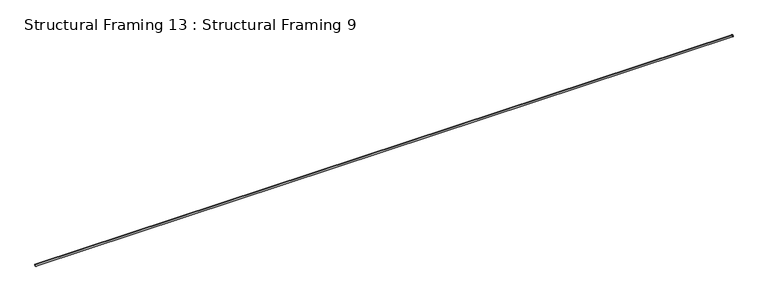
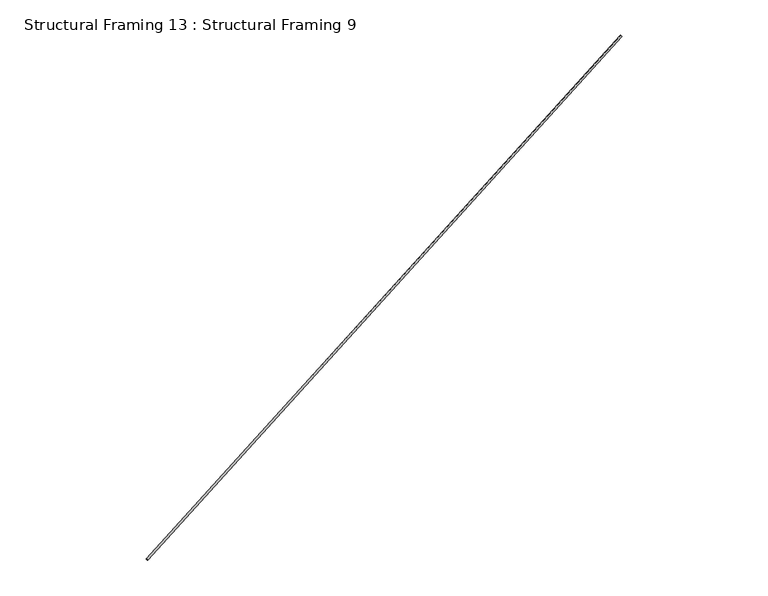
"""IFC4 building model written with IfcOpenShell, lengths in millimetres: beam geometry, Structural Framing 13 : Structural Framing 9."""

from ifc_helpers import new_model, si_unit, point, frame, origin, origin_2d, place, context, project, spatial, circle_curve, trimmed, segment, composite_curve, outline, extrude, source, transform, mapped, element, save


def structural_framing_13_structural_framing_9_8a389818(model_context):
    return source(origin(), model_context, "Body", "SweptSolid", [
        extrude(outline(composite_curve([segment(trimmed(circle_curve(origin_2d(), 6.35), [point((0.0, -6.35))], [point((0.0, 6.3499999))], False, "CARTESIAN"), True, "CONTINUOUS"), segment(trimmed(circle_curve(origin_2d(), 6.35), [point((0.0, 6.3499999))], [point((0.0, -6.35))], False, "CARTESIAN"), True, "CONTINUOUS")], self_intersect=False)), frame((23270.2350052, 2544.1506464, 2962.9722581), z_axis=(0.8890536510975653, 0.293078351767279, 0.35169402212074025), x_axis=(0.0, 0.7682212795973775, -0.640184399664478)), (0.0, 0.0, 1.0), 5574.8064179),
    ])


if __name__ == "__main__":
    model = new_model("IFC4")
    model_context = context("Model", 3, world=origin())
    ifc_project = project(units=[si_unit("LENGTHUNIT", "METRE", prefix="MILLI")], contexts=[model_context])
    site = spatial("IfcSite", under=ifc_project)
    building = spatial("IfcBuilding", under=site)
    placement = place(None, origin())
    structural_framing_13_structural_framing_9_shape = structural_framing_13_structural_framing_9_8a389818(model_context)
    element("IfcBeam", 1, ObjectType="Structural Framing 13 : Structural Framing 9", at=placement, inside=building, context=model_context, shape_type="MappedRepresentation", body=[
        mapped(structural_framing_13_structural_framing_9_shape, transform((0.0, 0.0, 0.0), x_axis=(1.0, 0.0, 0.0), y_axis=(0.0, 1.0, 0.0), z_axis=(0.0, 0.0, 1.0))),
    ])
    save(model, "model.ifc")

# Revit data of these elements
# Type "Structural Framing 13 : Structural Framing 9"
#   Structural Material [instance default] = EXISTING LATERAL BRACING (1/4" CABLE)
# Element 1 (IfcBeam, "Structural Framing 13 : Structural Framing 9")
#   Materials on its faces: "EXISTING LATERAL BRACING (1/4\" CABLE)"
# Materials
#   "EXISTING LATERAL BRACING (1/4\" CABLE)": class "Generic", colour RGB 120 120 120, transparency 0, Cost = 0
